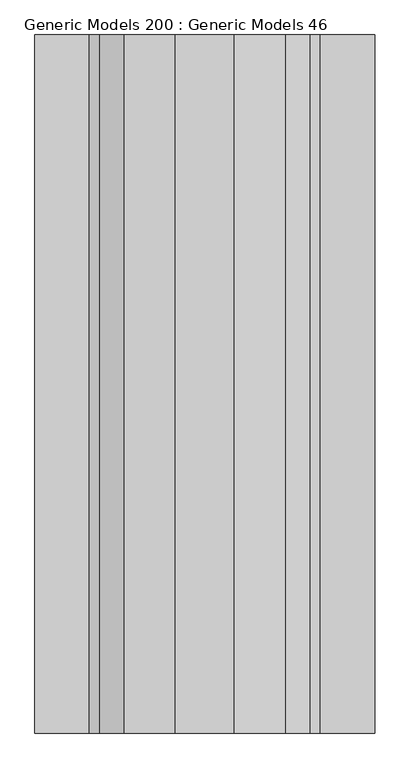
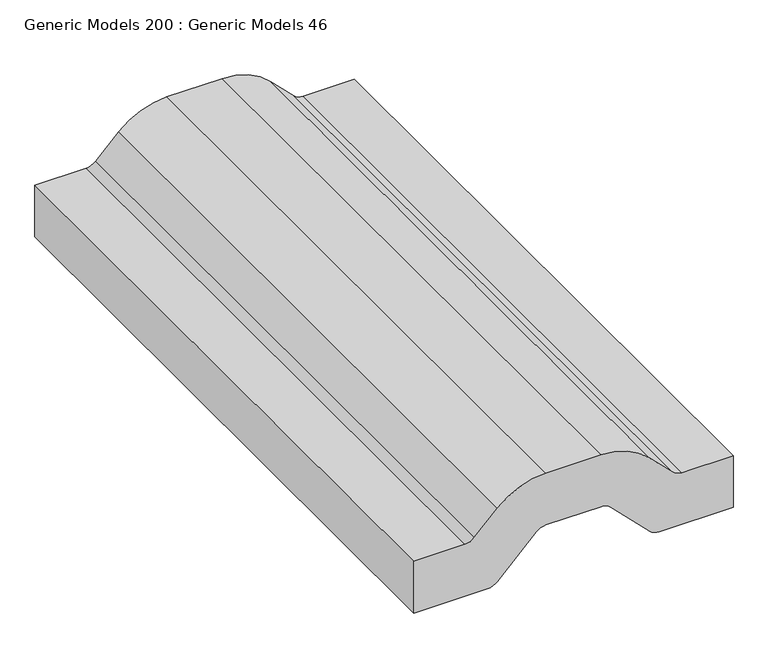
"""IFC4 building model written with IfcOpenShell, lengths in millimetres: proxy geometry, Generic Models 200 : Generic Models 46."""

from ifc_helpers import new_model, si_unit, point, frame, frame_2d, origin, place, context, project, spatial, polyline, circle_curve, trimmed, segment, composite_curve, outline, extrude, source, transform, mapped, element, save


def generic_models_200_generic_models_46_1dc11e6b(model_context):
    return source(origin(), model_context, "Body", "SweptSolid", [
        extrude(outline(composite_curve([segment(trimmed(circle_curve(frame_2d((238.3731772, 50217.3985863)), 25.4), [point((263.7731772, 50217.3985863))], [point((256.3336895, 50235.3590986))], True, "CARTESIAN"), True, "CONTINUOUS"), segment(polyline([(256.3336895, 50235.3590986), (183.9225951, 50307.7701929)]), True, "CONTINUOUS"), segment(trimmed(circle_curve(frame_2d((201.8831074, 50325.7307052)), 25.4), [point((183.9225951, 50307.7701929))], [point((176.4831074, 50325.7307052))], False, "CARTESIAN"), True, "CONTINUOUS"), segment(polyline([(176.4831074, 50325.7307052), (176.4831074, 50462.8696108), (278.0831074, 50462.8696108), (278.0831074, 50367.8148031)]), True, "CONTINUOUS"), segment(trimmed(circle_curve(frame_2d((303.4831074, 50367.8148031)), 25.4), [point((278.0831074, 50367.8148031))], [point((285.5225951, 50349.8542909))], True, "CARTESIAN"), True, "CONTINUOUS"), segment(polyline([(285.5225951, 50349.8542909), (328.1757385, 50307.2011475)]), True, "CONTINUOUS"), segment(trimmed(circle_curve(frame_2d((238.3731772, 50217.3985863)), 127.0), [point((328.1757385, 50307.2011475))], [point((365.3731772, 50217.3985863))], False, "CARTESIAN"), True, "CONTINUOUS"), segment(polyline([(365.3731772, 50217.3985863), (365.3731772, 50114.6156353)]), True, "CONTINUOUS"), segment(trimmed(circle_curve(frame_2d((238.3731772, 50114.6156353)), 127.0), [point((365.3731772, 50114.6156353))], [point((328.1757385, 50024.8130741))], False, "CARTESIAN"), True, "CONTINUOUS"), segment(polyline([(328.1757385, 50024.8130741), (285.5225951, 49982.1599308)]), True, "CONTINUOUS"), segment(trimmed(circle_curve(frame_2d((303.4831074, 49964.1994185)), 25.4), [point((285.5225951, 49982.1599308))], [point((278.0831074, 49964.1994185))], True, "CARTESIAN"), True, "CONTINUOUS"), segment(polyline([(278.0831074, 49964.1994185), (278.0831074, 49869.1446108), (176.4831074, 49869.1446108), (176.4831074, 50006.2835165)]), True, "CONTINUOUS"), segment(trimmed(circle_curve(frame_2d((201.8831074, 50006.2835165)), 25.4), [point((176.4831074, 50006.2835165))], [point((183.9225951, 50024.2440287))], False, "CARTESIAN"), True, "CONTINUOUS"), segment(polyline([(183.9225951, 50024.2440287), (256.3336895, 50096.6551231)]), True, "CONTINUOUS"), segment(trimmed(circle_curve(frame_2d((238.3731772, 50114.6156353)), 25.4), [point((256.3336895, 50096.6551231))], [point((263.7731772, 50114.6156353))], True, "CARTESIAN"), True, "CONTINUOUS"), segment(polyline([(263.7731772, 50114.6156353), (263.7731772, 50217.3985863)]), True, "CONTINUOUS")], self_intersect=False)), frame((0.0, 0.0, 0.0), z_axis=(0.0, 1.0, 0.0), x_axis=(0.0, 0.0, 1.0)), (0.0, 0.0, 1.0), 1219.2),
    ])


if __name__ == "__main__":
    model = new_model("IFC4")
    model_context = context("Model", 3, world=origin())
    ifc_project = project(units=[si_unit("LENGTHUNIT", "METRE", prefix="MILLI")], contexts=[model_context])
    site = spatial("IfcSite", under=ifc_project)
    building = spatial("IfcBuilding", under=site)
    placement = place(None, origin())
    generic_models_200_generic_models_46_shape = generic_models_200_generic_models_46_1dc11e6b(model_context)
    element("IfcBuildingElementProxy", 1, Name="Generic Models 200 : Generic Models 46", ObjectType="Generic Models 200 : Generic Models 46", at=placement, inside=building, context=model_context, shape_type="MappedRepresentation", body=[
        mapped(generic_models_200_generic_models_46_shape, transform((0.0, 0.0, 0.0), x_axis=(1.0, 0.0, 0.0), y_axis=(0.0, 1.0, 0.0), z_axis=(0.0, 0.0, 1.0))),
    ])
    save(model, "model.ifc")

# Revit data of these elements
# Element 1 (IfcBuildingElementProxy, "Generic Models 200 : Generic Models 46")
#   Materials on its faces: "BATT. INSULATION - EXTEND 4'-0\" MIN. - EACH SIDE OF STUD"
# Materials
#   "BATT. INSULATION - EXTEND 4'-0\" MIN. - EACH SIDE OF STUD": class "Unassigned", colour RGB 255 255 255, transparency 0, Cost = 0
